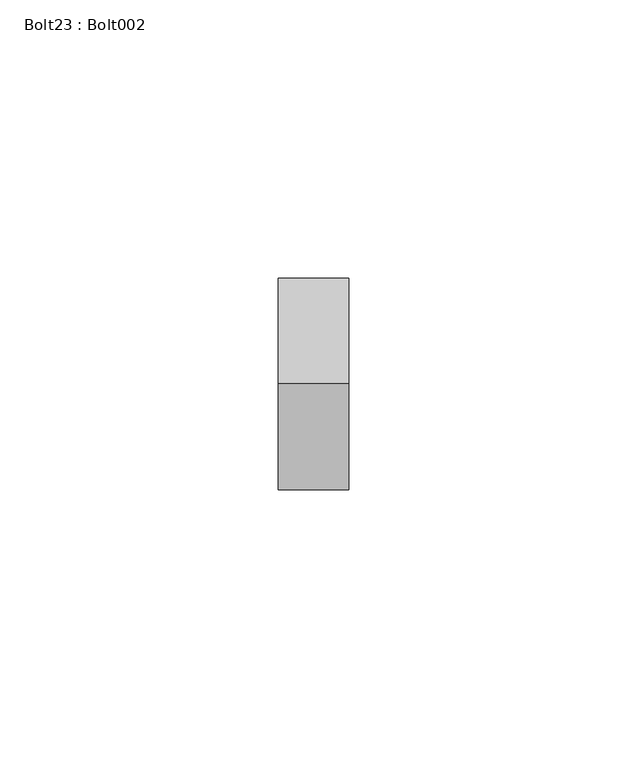
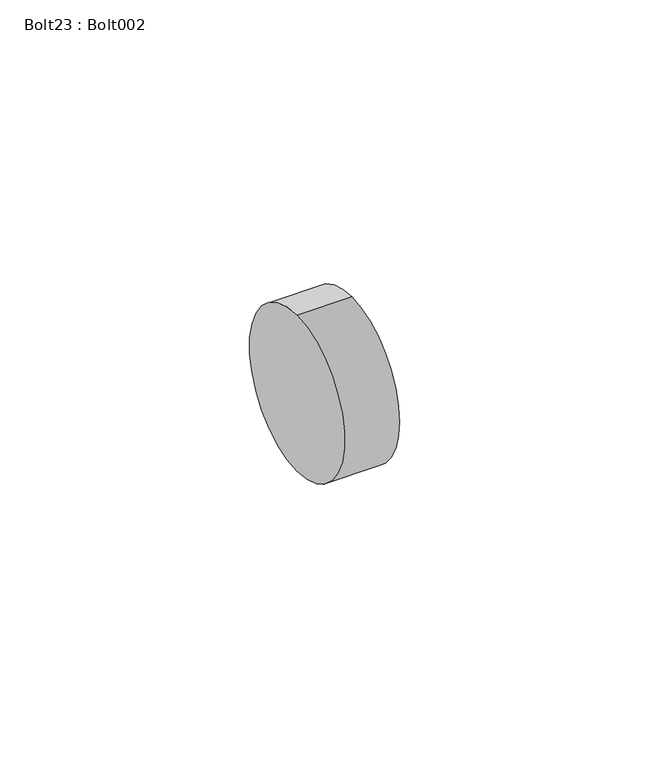
"""IFC4 building model written with IfcOpenShell, lengths in millimetres: proxy geometry, Bolt23 : Bolt002."""

from ifc_helpers import new_model, si_unit, point, frame, frame_2d, origin, place, context, project, spatial, circle_curve, trimmed, segment, composite_curve, outline, extrude, source, transform, mapped, element, save


def bolt23_bolt002_8e1fe756(model_context):
    return source(origin(), model_context, "Body", "SweptSolid", [
        extrude(outline(composite_curve([segment(trimmed(circle_curve(frame_2d((1985.8304801, 39960.0063132)), 19.05), [point((1985.8304801, 39979.0563132))], [point((1985.8304801, 39940.9563132))], False, "CARTESIAN"), True, "CONTINUOUS"), segment(trimmed(circle_curve(frame_2d((1985.8304801, 39960.0063132)), 19.05), [point((1985.8304801, 39940.9563132))], [point((1985.8304801, 39979.0563132))], False, "CARTESIAN"), True, "CONTINUOUS")], self_intersect=False)), frame((10268.2640809, 0.0, 0.0), z_axis=(1.0, 0.0, 0.0), x_axis=(0.0, 1.0, 0.0)), (0.0, 0.0, 1.0), 12.7),
    ])


if __name__ == "__main__":
    model = new_model("IFC4")
    model_context = context("Model", 3, world=origin())
    ifc_project = project(units=[si_unit("LENGTHUNIT", "METRE", prefix="MILLI")], contexts=[model_context])
    site = spatial("IfcSite", under=ifc_project)
    building = spatial("IfcBuilding", under=site)
    placement = place(None, origin())
    bolt23_bolt002_shape = bolt23_bolt002_8e1fe756(model_context)
    element("IfcBuildingElementProxy", 1, Name="Bolt23 : Bolt002", ObjectType="Bolt23 : Bolt002", at=placement, inside=building, context=model_context, shape_type="MappedRepresentation", body=[
        mapped(bolt23_bolt002_shape, transform((0.0, 0.0, 0.0), x_axis=(1.0, 0.0, 0.0), y_axis=(0.0, 1.0, 0.0), z_axis=(0.0, 0.0, 1.0))),
    ])
    save(model, "model.ifc")

# Revit data of these elements
# Type "Bolt23 : Bolt002"
#   NameOverride = "Bolt002"
# Element 1 (IfcBuildingElementProxy, "Bolt23 : Bolt002")
#   Materials on its faces: "TUBE STEEL STRINGER WELDED TO ANCHORED STEEL PLATE - SEE STRUCT DWGS"
# Materials
#   "TUBE STEEL STRINGER WELDED TO ANCHORED STEEL PLATE - SEE STRUCT DWGS": class "Unassigned", colour RGB 128 128 128, transparency 0, Cost = 0
